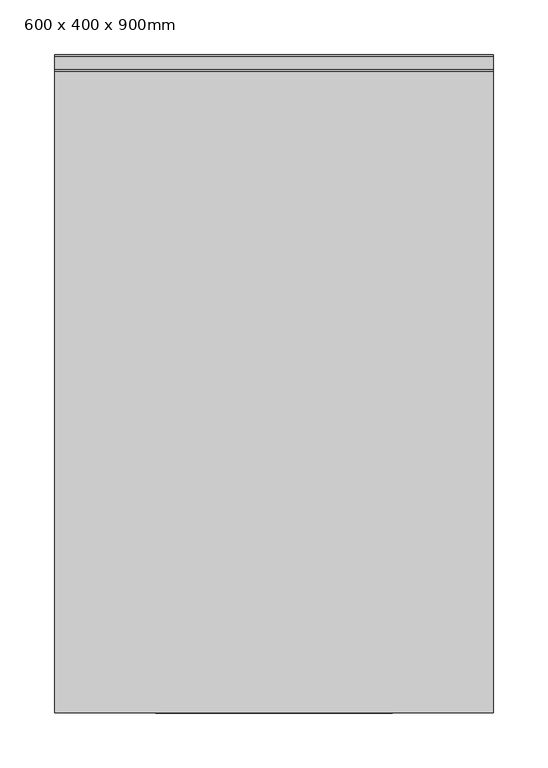
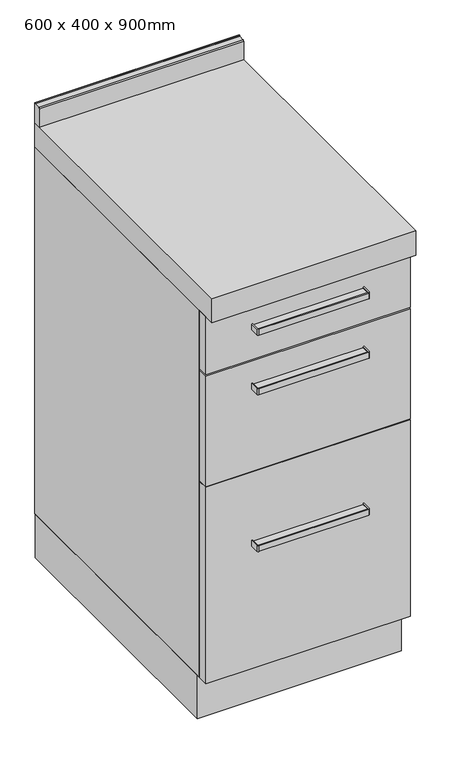
"""IFC4 building model written with IfcOpenShell, lengths in millimetres: furniture geometry, Küchenelement (1) - 2 Schubläden : 600 x 400 x 900mm."""

import ifcopenshell
import ifcopenshell.guid

model = None  # the IFC model being written
_history = None  # IfcOwnerHistory: only IFC2X3 demands one
_inside = {}  # id of a spatial element -> (the spatial element, [elements in it])
_under = {}  # id of a project, library or spatial element -> (it, [spatial elements below it])
_declared = {}  # id of a project -> (the project, [libraries it declares])
_typed = {}  # id of a type object -> (the type object, [elements of that type])
_made_of = {}  # id of a material, layer set ... -> (it, [elements and type objects made of it])


def new_model(schema):
    """Start an empty IFC model of exactly this schema.

    Asked for "IFC4X3", IfcOpenShell would pick the latest addendum, in which some entities
    have other attributes; the version numbers below select the first issue.
    IFC2X3 requires an IfcOwnerHistory on every rooted entity: one is made here for all.
    """
    global model, _history
    if schema == "IFC4X3":
        model = ifcopenshell.file(schema_version=(4, 3, 0, 0))
    else:
        model = ifcopenshell.file(schema=schema)
    _inside.clear()
    _under.clear()
    _declared.clear()
    _typed.clear()
    _made_of.clear()
    _history = None
    if model.schema == "IFC2X3":
        org = make("IfcOrganization", Name="unknown")
        user = make(
            "IfcPersonAndOrganization",
            ThePerson=make("IfcPerson", FamilyName="unknown"),
            TheOrganization=org,
        )
        app = make(
            "IfcApplication",
            ApplicationDeveloper=org,
            Version="unknown",
            ApplicationFullName="unknown",
            ApplicationIdentifier="unknown",
        )
        _history = make(
            "IfcOwnerHistory",
            OwningUser=user,
            OwningApplication=app,
            ChangeAction="ADDED",
            CreationDate=0,
        )
    return model


def make(cls, **values):
    """One entity of the class cls with the attributes given. An attribute that is None is left unset."""
    return model.create_entity(
        cls, **{name: value for name, value in values.items() if value is not None}
    )


def rooted(cls, **values):
    """An entity with a GlobalId (a new one), such as an element, a storey or a relation."""
    return make(cls, GlobalId=ifcopenshell.guid.new(), OwnerHistory=_history, **values)


def si_unit(unit_type, name, prefix=None):
    """IfcSIUnit, for example si_unit("LENGTHUNIT", "METRE", prefix="MILLI")."""
    return make("IfcSIUnit", UnitType=unit_type, Prefix=prefix, Name=name)


def assignment(units):
    """IfcUnitAssignment: the units of a project."""
    return None if units is None else make("IfcUnitAssignment", Units=units)


def point(xyz):
    """IfcCartesianPoint."""
    return None if xyz is None else make("IfcCartesianPoint", Coordinates=xyz)


def direction(xyz):
    """IfcDirection."""
    return None if xyz is None else make("IfcDirection", DirectionRatios=xyz)


def frame(location, z_axis=None, x_axis=None):
    """IfcAxis2Placement3D, a coordinate frame: its origin and axes. An axis left out is left unset."""
    return make(
        "IfcAxis2Placement3D",
        Location=point(location),
        Axis=direction(z_axis),
        RefDirection=direction(x_axis),
    )


def frame_2d(location, x_axis=None):
    """IfcAxis2Placement2D, a coordinate frame in the plane: its origin and x axis."""
    return make(
        "IfcAxis2Placement2D", Location=point(location), RefDirection=direction(x_axis)
    )


def origin():
    """The frame at (0, 0, 0) with its axes left unset."""
    return frame((0.0, 0.0, 0.0))


def origin_with_axes():
    """The frame at (0, 0, 0) with the z axis (0, 0, 1) and the x axis (1, 0, 0) written out."""
    return frame((0.0, 0.0, 0.0), z_axis=(0.0, 0.0, 1.0), x_axis=(1.0, 0.0, 0.0))


def place(relative_to, where):
    """IfcLocalPlacement: puts the frame where relative to a parent placement (None: the world)."""
    return make(
        "IfcLocalPlacement", PlacementRelTo=relative_to, RelativePlacement=where
    )


def context(
    kind, dimensions, precision=None, world=None, true_north=None, identifier=None
):
    """IfcGeometricRepresentationContext, for example the 3D "Model" context."""
    return make(
        "IfcGeometricRepresentationContext",
        ContextIdentifier=identifier,
        ContextType=kind,
        CoordinateSpaceDimension=dimensions,
        Precision=precision,
        WorldCoordinateSystem=world,
        TrueNorth=true_north,
    )


def project(units=None, contexts=None):
    """IfcProject with its units and contexts."""
    return rooted(
        "IfcProject",
        Name="project",
        RepresentationContexts=contexts,
        UnitsInContext=assignment(units),
    )


def spatial(cls, under=None, at=None, **own):
    """A site, building, storey or space (cls), placed at a placement, below another one or the project."""
    s = rooted(cls, ObjectPlacement=at, **own)
    if under is not None:
        _under.setdefault(under.id(), (under, []))[1].append(s)
    return s


def polyline(points):
    """IfcPolyline through the points."""
    return make("IfcPolyline", Points=[point(p) for p in points])


def circle_curve(where, radius):
    """IfcCircle in the frame where."""
    return make("IfcCircle", Position=where, Radius=radius)


def trimmed(basis, trim1, trim2, sense, master):
    """IfcTrimmedCurve: the piece of a basis curve between two trims."""
    return make(
        "IfcTrimmedCurve",
        BasisCurve=basis,
        Trim1=trim1,
        Trim2=trim2,
        SenseAgreement=sense,
        MasterRepresentation=master,
    )


def segment(curve, same_sense, transition):
    """IfcCompositeCurveSegment."""
    return make(
        "IfcCompositeCurveSegment",
        Transition=transition,
        SameSense=same_sense,
        ParentCurve=curve,
    )


def composite_curve(segments, self_intersect=None):
    """IfcCompositeCurve: segments joined end to end."""
    return make("IfcCompositeCurve", Segments=segments, SelfIntersect=self_intersect)


def outline(outer, holes=None, kind="AREA"):
    """IfcArbitraryClosedProfileDef: a profile drawn as a closed curve; with holes, ...WithVoids."""
    if holes is None:
        return make("IfcArbitraryClosedProfileDef", ProfileType=kind, OuterCurve=outer)
    return make(
        "IfcArbitraryProfileDefWithVoids",
        ProfileType=kind,
        OuterCurve=outer,
        InnerCurves=holes,
    )


def extrude(swept, where, along, depth):
    """IfcExtrudedAreaSolid: the profile swept, set in the frame where, extruded along a direction by depth."""
    return make(
        "IfcExtrudedAreaSolid",
        SweptArea=swept,
        Position=where,
        ExtrudedDirection=direction(along),
        Depth=depth,
    )


def shape(context_of_items, identifier, shape_type, items):
    """IfcShapeRepresentation: the items that make up one representation, for example the "Body"."""
    return make(
        "IfcShapeRepresentation",
        ContextOfItems=context_of_items,
        RepresentationIdentifier=identifier,
        RepresentationType=shape_type,
        Items=items,
    )


def source(mapping_origin, context_of_items, identifier, shape_type, items):
    """IfcRepresentationMap: a shape defined once, which mapped items show again and again."""
    return make(
        "IfcRepresentationMap",
        MappingOrigin=mapping_origin,
        MappedRepresentation=shape(context_of_items, identifier, shape_type, items),
    )


def transform(
    local_origin,
    x_axis=None,
    y_axis=None,
    z_axis=None,
    scale=None,
    scale2=None,
    scale3=None,
    uniform=True,
):
    """IfcCartesianTransformationOperator3D, or its non-uniform kind. x_axis, y_axis, z_axis: its Axis1, 2, 3."""
    if uniform:
        return make(
            "IfcCartesianTransformationOperator3D",
            Axis1=direction(x_axis),
            Axis2=direction(y_axis),
            LocalOrigin=point(local_origin),
            Scale=scale,
            Axis3=direction(z_axis),
        )
    return make(
        "IfcCartesianTransformationOperator3DnonUniform",
        Axis1=direction(x_axis),
        Axis2=direction(y_axis),
        LocalOrigin=point(local_origin),
        Scale=scale,
        Axis3=direction(z_axis),
        Scale2=scale2,
        Scale3=scale3,
    )


def mapped(mapping_source, mapping_target):
    """IfcMappedItem: shows the shape of a source again, moved by a transform."""
    return make(
        "IfcMappedItem", MappingSource=mapping_source, MappingTarget=mapping_target
    )


def made_of(thing, what):
    """Note that an element or type object is made of a material, layer set ...; save() writes the relation."""
    if what is not None:
        _made_of.setdefault(what.id(), (what, []))[1].append(thing)
    return thing


def element(
    cls,
    number,
    at=None,
    inside=None,
    cuts=None,
    type_object=None,
    material=None,
    context=None,
    identifier="Body",
    shape_type=None,
    held_by="IfcProductDefinitionShape",
    body=None,
    shapes=None,
    **own,
):
    """One element of the class cls, such as IfcWall. Its Tag is "e" and its number.

    at: its placement. inside: the storey or other place that contains it. cuts: it is an
    opening in that element (IfcRelVoidsElement). A single representation is given by context,
    identifier, shape_type and body (its items); several are given by shapes. held_by: the class
    of the entity that holds the representations. save() writes the other relations.
    """
    e = rooted(cls, Tag="e%d" % number, ObjectPlacement=at, **own)
    if body is not None:
        shapes = [shape(context, identifier, shape_type, body)]
    if shapes is not None:
        e.Representation = make(held_by, Representations=shapes)
    if inside is not None:
        _inside.setdefault(inside.id(), (inside, []))[1].append(e)
    if cuts is not None:
        rooted(
            "IfcRelVoidsElement", RelatingBuildingElement=cuts, RelatedOpeningElement=e
        )
    if type_object is not None:
        _typed.setdefault(type_object.id(), (type_object, []))[1].append(e)
    return made_of(e, material)


def aggregate(whole, parts):
    """IfcRelAggregates: a whole, such as a stair, and the parts it consists of."""
    return rooted("IfcRelAggregates", RelatingObject=whole, RelatedObjects=parts)


def save(model, path):
    """Write the relations noted so far, then the file.

    IfcRelAggregates (storeys below a building ...), IfcRelContainedInSpatialStructure (elements
    in a storey), IfcRelDefinesByType, IfcRelAssociatesMaterial and IfcRelDeclares: one each for
    every whole, place, type object, material and project.
    """
    for whole, parts in _under.values():
        aggregate(whole, parts)
    for where, things in _inside.values():
        rooted(
            "IfcRelContainedInSpatialStructure",
            RelatedElements=things,
            RelatingStructure=where,
        )
    for kind, things in _typed.values():
        rooted("IfcRelDefinesByType", RelatedObjects=things, RelatingType=kind)
    for what, things in _made_of.values():
        rooted("IfcRelAssociatesMaterial", RelatedObjects=things, RelatingMaterial=what)
    for by, libraries in _declared.values():
        rooted("IfcRelDeclares", RelatingContext=by, RelatedDefinitions=libraries)
    model.write(path)


def furniture_600_x_400_x_900mm_10b2b102(model_context):
    return source(origin(), model_context, "Body", "SweptSolid", [
        extrude(outline(composite_curve([segment(polyline([(-63.2996736, -577.0), (152.7003264, -577.0), (152.7003264, -597.5)]), True, "CONTINUOUS"), segment(trimmed(circle_curve(frame_2d((152.2003264, -597.5)), 0.5), [point((152.7003264, -597.5))], [point((152.2003264, -598.0))], False, "CARTESIAN"), True, "CONTINUOUS"), segment(polyline([(152.2003264, -598.0), (-62.7996736, -598.0)]), True, "CONTINUOUS"), segment(trimmed(circle_curve(frame_2d((-62.7996736, -597.5)), 0.5), [point((-62.7996736, -598.0))], [point((-63.2996736, -597.5))], False, "CARTESIAN"), True, "CONTINUOUS"), segment(polyline([(-63.2996736, -597.5), (-63.2996736, -577.0)]), True, "CONTINUOUS")], self_intersect=False)), frame((0.0, 0.0, 346.445389), z_axis=(0.0, 0.0, 1.0), x_axis=(1.0, 0.0, 0.0)), (0.0, 0.0, 1.0), 6.4890959),
        extrude(outline(composite_curve([segment(polyline([(-65.2996736, -577.0), (-63.2996736, -577.0), (-63.2996736, -597.5)]), True, "CONTINUOUS"), segment(trimmed(circle_curve(frame_2d((-62.7996736, -597.5)), 0.5), [point((-63.2996736, -597.5))], [point((-62.7996736, -598.0))], True, "CARTESIAN"), True, "CONTINUOUS"), segment(polyline([(-62.7996736, -598.0), (152.2003264, -598.0)]), True, "CONTINUOUS"), segment(trimmed(circle_curve(frame_2d((152.2003264, -597.5)), 0.5), [point((152.2003264, -598.0))], [point((152.7003264, -597.5))], True, "CARTESIAN"), True, "CONTINUOUS"), segment(polyline([(152.7003264, -597.5), (152.7003264, -577.0), (154.7003264, -577.0), (154.7003264, -597.5)]), True, "CONTINUOUS"), segment(trimmed(circle_curve(frame_2d((152.2003264, -597.5)), 2.5), [point((154.7003264, -597.5))], [point((152.2003264, -600.0))], False, "CARTESIAN"), True, "CONTINUOUS"), segment(polyline([(152.2003264, -600.0), (-62.7996736, -600.0)]), True, "CONTINUOUS"), segment(trimmed(circle_curve(frame_2d((-62.7996736, -597.5)), 2.5), [point((-62.7996736, -600.0))], [point((-65.2996736, -597.5))], False, "CARTESIAN"), True, "CONTINUOUS"), segment(polyline([(-65.2996736, -597.5), (-65.2996736, -577.0)]), True, "CONTINUOUS")], self_intersect=False)), frame((0.0, 0.0, 343.68), z_axis=(0.0, 0.0, 1.0), x_axis=(1.0, 0.0, 0.0)), (0.0, 0.0, 1.0), 12.0),
        extrude(outline(composite_curve([segment(polyline([(-63.2996736, -577.0), (152.7003264, -577.0), (152.7003264, -597.5)]), True, "CONTINUOUS"), segment(trimmed(circle_curve(frame_2d((152.2003264, -597.5)), 0.5), [point((152.7003264, -597.5))], [point((152.2003264, -598.0))], False, "CARTESIAN"), True, "CONTINUOUS"), segment(polyline([(152.2003264, -598.0), (-62.7996736, -598.0)]), True, "CONTINUOUS"), segment(trimmed(circle_curve(frame_2d((-62.7996736, -597.5)), 0.5), [point((-62.7996736, -598.0))], [point((-63.2996736, -597.5))], False, "CARTESIAN"), True, "CONTINUOUS"), segment(polyline([(-63.2996736, -597.5), (-63.2996736, -577.0)]), True, "CONTINUOUS")], self_intersect=False)), frame((0.0, 0.0, 671.435389), z_axis=(0.0, 0.0, 1.0), x_axis=(1.0, 0.0, 0.0)), (0.0, 0.0, 1.0), 6.4890959),
        extrude(outline(composite_curve([segment(polyline([(-65.2996736, -577.0), (-63.2996736, -577.0), (-63.2996736, -597.5)]), True, "CONTINUOUS"), segment(trimmed(circle_curve(frame_2d((-62.7996736, -597.5)), 0.5), [point((-63.2996736, -597.5))], [point((-62.7996736, -598.0))], True, "CARTESIAN"), True, "CONTINUOUS"), segment(polyline([(-62.7996736, -598.0), (152.2003264, -598.0)]), True, "CONTINUOUS"), segment(trimmed(circle_curve(frame_2d((152.2003264, -597.5)), 0.5), [point((152.2003264, -598.0))], [point((152.7003264, -597.5))], True, "CARTESIAN"), True, "CONTINUOUS"), segment(polyline([(152.7003264, -597.5), (152.7003264, -577.0), (154.7003264, -577.0), (154.7003264, -597.5)]), True, "CONTINUOUS"), segment(trimmed(circle_curve(frame_2d((152.2003264, -597.5)), 2.5), [point((154.7003264, -597.5))], [point((152.2003264, -600.0))], False, "CARTESIAN"), True, "CONTINUOUS"), segment(polyline([(152.2003264, -600.0), (-62.7996736, -600.0)]), True, "CONTINUOUS"), segment(trimmed(circle_curve(frame_2d((-62.7996736, -597.5)), 2.5), [point((-62.7996736, -600.0))], [point((-65.2996736, -597.5))], False, "CARTESIAN"), True, "CONTINUOUS"), segment(polyline([(-65.2996736, -597.5), (-65.2996736, -577.0)]), True, "CONTINUOUS")], self_intersect=False)), frame((0.0, 0.0, 668.67), z_axis=(0.0, 0.0, 1.0), x_axis=(1.0, 0.0, 0.0)), (0.0, 0.0, 1.0), 12.0),
        extrude(outline(composite_curve([segment(polyline([(-63.2996736, -577.0), (152.7003264, -577.0), (152.7003264, -597.5)]), True, "CONTINUOUS"), segment(trimmed(circle_curve(frame_2d((152.2003264, -597.5)), 0.5), [point((152.7003264, -597.5))], [point((152.2003264, -598.0))], False, "CARTESIAN"), True, "CONTINUOUS"), segment(polyline([(152.2003264, -598.0), (-62.7996736, -598.0)]), True, "CONTINUOUS"), segment(trimmed(circle_curve(frame_2d((-62.7996736, -597.5)), 0.5), [point((-62.7996736, -598.0))], [point((-63.2996736, -597.5))], False, "CARTESIAN"), True, "CONTINUOUS"), segment(polyline([(-63.2996736, -597.5), (-63.2996736, -577.0)]), True, "CONTINUOUS")], self_intersect=False)), frame((0.0, 0.0, 794.465389), z_axis=(0.0, 0.0, 1.0), x_axis=(1.0, 0.0, 0.0)), (0.0, 0.0, 1.0), 6.4890959),
        extrude(outline(composite_curve([segment(polyline([(-65.2996736, -577.0), (-63.2996736, -577.0), (-63.2996736, -597.5)]), True, "CONTINUOUS"), segment(trimmed(circle_curve(frame_2d((-62.7996736, -597.5)), 0.5), [point((-63.2996736, -597.5))], [point((-62.7996736, -598.0))], True, "CARTESIAN"), True, "CONTINUOUS"), segment(polyline([(-62.7996736, -598.0), (152.2003264, -598.0)]), True, "CONTINUOUS"), segment(trimmed(circle_curve(frame_2d((152.2003264, -597.5)), 0.5), [point((152.2003264, -598.0))], [point((152.7003264, -597.5))], True, "CARTESIAN"), True, "CONTINUOUS"), segment(polyline([(152.7003264, -597.5), (152.7003264, -577.0), (154.7003264, -577.0), (154.7003264, -597.5)]), True, "CONTINUOUS"), segment(trimmed(circle_curve(frame_2d((152.2003264, -597.5)), 2.5), [point((154.7003264, -597.5))], [point((152.2003264, -600.0))], False, "CARTESIAN"), True, "CONTINUOUS"), segment(polyline([(152.2003264, -600.0), (-62.7996736, -600.0)]), True, "CONTINUOUS"), segment(trimmed(circle_curve(frame_2d((-62.7996736, -597.5)), 2.5), [point((-62.7996736, -600.0))], [point((-65.2996736, -597.5))], False, "CARTESIAN"), True, "CONTINUOUS"), segment(polyline([(-65.2996736, -597.5), (-65.2996736, -577.0)]), True, "CONTINUOUS")], self_intersect=False)), frame((0.0, 0.0, 791.7), z_axis=(0.0, 0.0, 1.0), x_axis=(1.0, 0.0, 0.0)), (0.0, 0.0, 1.0), 12.0),
        extrude(outline(polyline([(244.7003264, -580.0), (-155.2996736, -580.0), (-155.2996736, -558.0), (244.7003264, -558.0), (244.7003264, -580.0)])), frame((0.0, 0.0, 730.0), z_axis=(0.0, 0.0, 1.0), x_axis=(1.0, 0.0, 0.0)), (0.0, 0.0, 1.0), 120.0),
        extrude(outline(polyline([(244.7003264, -580.0), (-155.2996736, -580.0), (-155.2996736, -558.0), (244.7003264, -558.0), (244.7003264, -580.0)])), frame((0.0, 0.0, 498.5), z_axis=(0.0, 0.0, 1.0), x_axis=(1.0, 0.0, 0.0)), (0.0, 0.0, 1.0), 228.5),
        extrude(outline(polyline([(244.7003264, -580.0), (-155.2996736, -580.0), (-155.2996736, -558.0), (244.7003264, -558.0), (244.7003264, -580.0)])), frame((0.0, 0.0, 90.0), z_axis=(0.0, 0.0, 1.0), x_axis=(1.0, 0.0, 0.0)), (0.0, 0.0, 1.0), 406.5),
        extrude(outline(composite_curve([segment(polyline([(0.0, 942.0034681), (0.0, 900.0), (-15.0, 900.0), (-15.0, 938.0)]), True, "CONTINUOUS"), segment(trimmed(circle_curve(frame_2d((-13.0, 938.0)), 2.0), [point((-15.0, 938.0))], [point((-13.0, 940.0))], False, "CARTESIAN"), True, "CONTINUOUS"), segment(polyline([(-13.0, 940.0), (-1.50449, 940.0), (-1.50449, 942.0034681), (0.0, 942.0034681)]), True, "CONTINUOUS")], self_intersect=False)), frame((-155.2996736, 0.0, 0.0), z_axis=(1.0, 0.0, 0.0), x_axis=(0.0, 1.0, 0.0)), (0.0, 0.0, 1.0), 400.0),
        extrude(outline(polyline([(244.7003264, -0.533703), (244.7003264, -550.533703), (-155.2996736, -550.533703), (-155.2996736, -0.533703), (244.7003264, -0.533703)])), origin_with_axes(), (0.0, 0.0, 1.0), 90.0),
        extrude(outline(polyline([(244.7003264, 0.0), (244.7003264, -600.0), (-155.2996736, -600.0), (-155.2996736, 0.0), (244.7003264, 0.0)])), frame((0.0, 0.0, 850.0), z_axis=(0.0, 0.0, 1.0), x_axis=(1.0, 0.0, 0.0)), (0.0, 0.0, 1.0), 50.0),
        extrude(outline(polyline([(244.7003264, 0.0), (244.7003264, -558.0), (222.7003264, -558.0), (222.7003264, -22.0), (-133.2996736, -22.0), (-133.2996736, -558.0), (-155.2996736, -558.0), (-155.2996736, 0.0), (244.7003264, 0.0)])), frame((0.0, 0.0, 90.0), z_axis=(0.0, 0.0, 1.0), x_axis=(1.0, 0.0, 0.0)), (0.0, 0.0, 1.0), 760.0),
    ])


if __name__ == "__main__":
    model = new_model("IFC4")
    model_context = context("Model", 3, world=origin())
    ifc_project = project(units=[si_unit("LENGTHUNIT", "METRE", prefix="MILLI")], contexts=[model_context])
    site = spatial("IfcSite", under=ifc_project)
    building = spatial("IfcBuilding", under=site)
    placement = place(None, origin())
    furniture_600_x_400_x_900mm_shape = furniture_600_x_400_x_900mm_10b2b102(model_context)
    element("IfcFurniture", 1, ObjectType="Küchenelement (1) - 2 Schubläden : 600 x 400 x 900mm", at=placement, inside=building, context=model_context, shape_type="MappedRepresentation", body=[
        mapped(furniture_600_x_400_x_900mm_shape, transform((0.0, 0.0, 0.0), x_axis=(1.0, 0.0, 0.0), y_axis=(0.0, 1.0, 0.0), z_axis=(0.0, 0.0, 1.0))),
    ])
    save(model, "model.ifc")

# Revit data of these elements
# Type "Küchenelement (1) - 2 Schubläden : 600 x 400 x 900mm"
#   Assembly Code = "C1030400"
#   Länge 3 = 0.12303 m
#   Länge 2 = 0.32499 m
#   Länge 1 = 0.35568 m
#   Depth = 0.600 m
#   Height = 0.900 m
#   Width = 0.400 m
#   1 = 0.000 m
#   Obermaterial = none
#   Material = none
#   Griffmaterial = none
# Element 1 (IfcFurniture, "Küchenelement (1) - 2 Schubläden : 600 x 400 x 900mm")
#   Materials on its faces: "Holz - Birke"
# Materials
#   "Holz - Birke": class "Holz", colour RGB 213 164 103, transparency 0, Cost = 0
